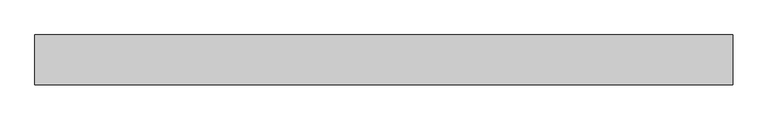
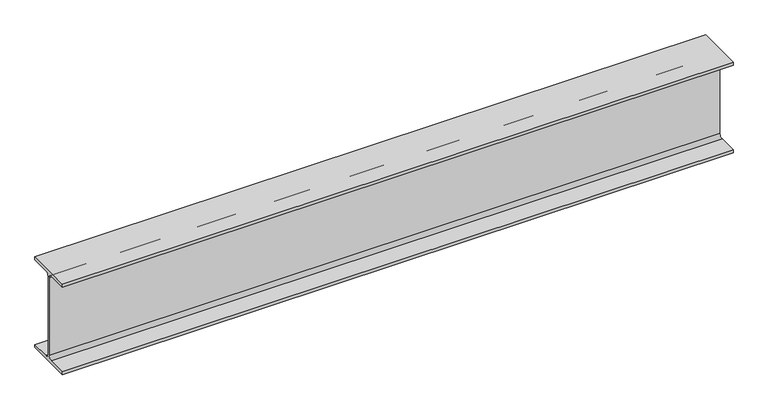
"""IFC4 building model written with IfcOpenShell, lengths in millimetres: beam geometry, 0912_Steel Framing_H-KSD3502 : H_SB_ASB_H-350x175x7x11."""

from ifc_helpers import new_model, si_unit, point, frame, frame_2d, origin, place, context, project, spatial, polyline, circle_curve, trimmed, segment, composite_curve, outline, extrude, source, transform, mapped, element, save


def beam_c9532cb6(model_context):
    return source(origin(), model_context, "Body", "SweptSolid", [
        extrude(outline(composite_curve([segment(polyline([(87.5, -164.0), (87.5, -175.0), (-87.5, -175.0), (-87.5, -164.0), (-17.5, -164.0)]), True, "CONTINUOUS"), segment(trimmed(circle_curve(frame_2d((-17.5, -150.0)), 14.0), [point((-17.5, -164.0))], [point((-3.5, -150.0))], True, "CARTESIAN"), True, "CONTINUOUS"), segment(polyline([(-3.5, -150.0), (-3.5, 150.0)]), True, "CONTINUOUS"), segment(trimmed(circle_curve(frame_2d((-17.5, 150.0)), 14.0), [point((-3.5, 150.0))], [point((-17.5, 164.0))], True, "CARTESIAN"), True, "CONTINUOUS"), segment(polyline([(-17.5, 164.0), (-87.5, 164.0), (-87.5, 175.0), (87.5, 175.0), (87.5, 164.0), (17.5, 164.0)]), True, "CONTINUOUS"), segment(trimmed(circle_curve(frame_2d((17.5, 150.0)), 14.0), [point((17.5, 164.0))], [point((3.5, 150.0))], True, "CARTESIAN"), True, "CONTINUOUS"), segment(polyline([(3.5, 150.0), (3.5, -150.0)]), True, "CONTINUOUS"), segment(trimmed(circle_curve(frame_2d((17.5, -150.0)), 14.0), [point((3.5, -150.0))], [point((17.5, -164.0))], True, "CARTESIAN"), True, "CONTINUOUS"), segment(polyline([(17.5, -164.0), (87.5, -164.0)]), True, "CONTINUOUS")], self_intersect=False)), frame((-1295.7739051, 0.0, 0.0), z_axis=(1.0, 0.0, 0.0), x_axis=(0.0, 1.0, 0.0)), (0.0, 0.0, 1.0), 2456.2874909),
    ])


if __name__ == "__main__":
    model = new_model("IFC4")
    model_context = context("Model", 3, world=origin())
    ifc_project = project(units=[si_unit("LENGTHUNIT", "METRE", prefix="MILLI")], contexts=[model_context])
    site = spatial("IfcSite", under=ifc_project)
    building = spatial("IfcBuilding", under=site)
    placement = place(None, origin())
    beam_shape = beam_c9532cb6(model_context)
    element("IfcBeam", 1, ObjectType="0912_Steel Framing_H-KSD3502 : H_SB_ASB_H-350x175x7x11", at=placement, inside=building, context=model_context, shape_type="MappedRepresentation", body=[
        mapped(beam_shape, transform((0.0, 0.0, 0.0), x_axis=(1.0, 0.0, 0.0), y_axis=(0.0, 1.0, 0.0), z_axis=(0.0, 0.0, 1.0))),
    ])
    save(model, "model.ifc")

# Revit data of these elements
# Type "0912_Steel Framing_H-KSD3502 : H_SB_ASB_H-350x175x7x11"
#   H_WM Code_1 = "S01AA002-00001 | Main Steel Structure Fabrication Work | Shelter/Building | Medium Steel - Standard (90KG/M>Weight≥30KG/M) | Material: (   )"
#   H_WM Code_2 = "S03AA028-00001 | Main Steel Structure Erection Work | Shelter/Building | Medium Steel (90KG/M>Weight≥30KG/M) | Material: (   )"
#   H_WM Code_3 = "S01AA010-00001 | Main Steel Structure Fabrication Work | Shelter/Building | Steel Painting/Coating | for Non-Fireproofed Steel Surface, Surface Preparation, Primer, Second & Final Coat | Material: (   )"
#   H_Q'ty Cal Type Tag = "SB-Q2"
#   Width = 17.5 cm
#   Web Thickness = 0.7 cm
#   Web Fillet = 1.4 cm
#   Warping Constant = 282000.0 cm⁶
#   W = 0
#   Torsional Moment of Inertia = 19.4042 cm⁴
#   Section Area = 63.14 cm²
#   Plastic Modulus weak axis = 174.0 cm³
#   Plastic Modulus strong axis = 868.0 cm³
#   Perimeter = 1.36 m²/m
#   Nominal Weight = 49.60 kgf/m
#   Moment of Inertia weak axis = 984.00 cm⁴
#   Moment of Inertia strong axis = 13600.00 cm⁴
#   Height = 35.0 cm
#   Flange Thickness = 1.1 cm
#   Elastic Modulus weak axis = 112.0 cm³
#   Elastic Modulus strong axis = 775.0 cm³
#   Centroid Vertical = 17.5 cm
#   Centroid Horizontal = 8.75 cm
#   Ix = 136000000
#   Length [instance default] = 1.5240 m
#   Zx = 868000
#   b = 0.1750 m
#   h = 0.3500 m
#   r = 0.0140 m
#   s = 0.0070 m
#   t = 0.0110 m
#   A = 0.006314 m²
#   Structural Material [instance default] = Steel, 45-345
#   Assembly Code = ""
# Element 1 (IfcBeam, "0912_Steel Framing_H-KSD3502 : H_SB_ASB_H-350x175x7x11")
#   Structural Material = none
# Materials
#   "Steel, 45-345": class "Metal", colour RGB 189 187 185, transparency 0, Description = "Steel 345 MPa", Cost = 0
